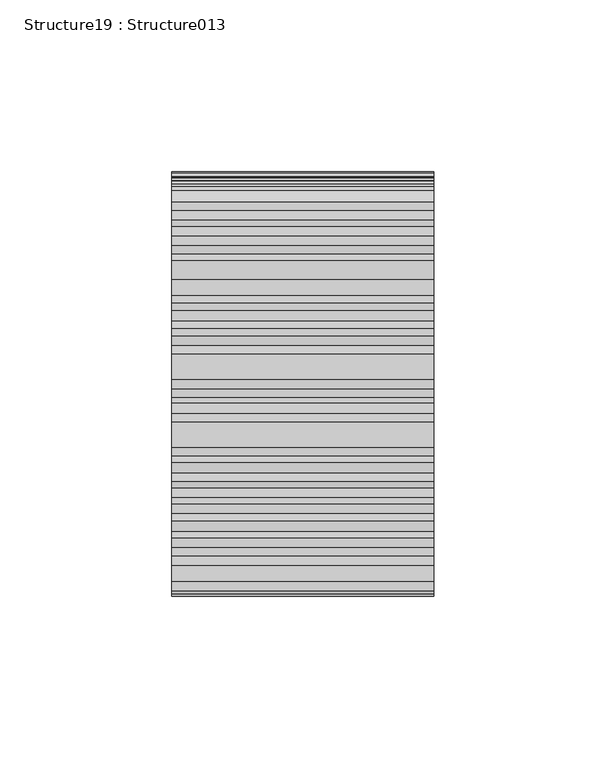
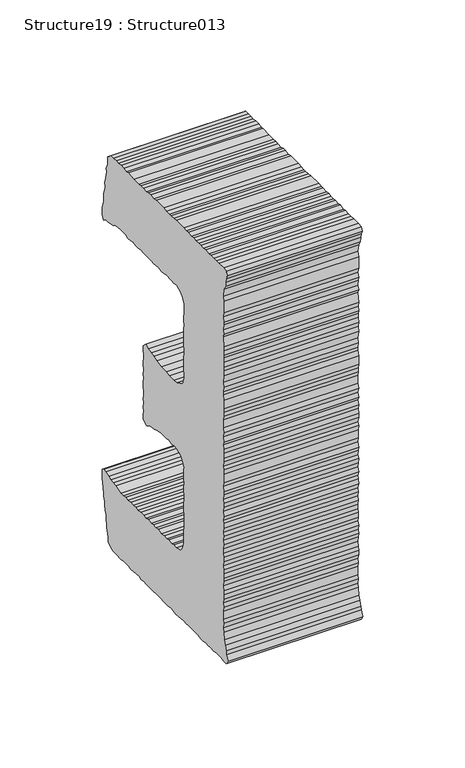
"""IFC4 building model written with IfcOpenShell, lengths in millimetres: proxy geometry, Structure19 : Structure013."""

from ifc_helpers import new_model, si_unit, frame, origin, place, context, project, spatial, polyline, outline, extrude, source, transform, mapped, element, save


def structure19_structure013_5d5198df(model_context):
    return source(origin(), model_context, "Body", "SweptSolid", [
        extrude(outline(polyline([(3.520981, 0.0), (5.3687336, -0.6528764), (7.3730967, -2.6179514), (11.6549807, -5.1627133), (12.9785054, -6.9870238), (17.377171, -10.4155139), (19.218173, -11.0577579), (21.470001, -13.2028271), (23.2331492, -14.9798898), (25.1815783, -16.4985708), (27.2738182, -17.3366394), (28.8385579, -19.3489622), (30.9822906, -20.6170736), (36.8382689, -25.1814496), (38.1096325, -26.5751964), (42.0165135, -29.6203706), (44.5911834, -30.8344637), (46.1186982, -32.4149751), (48.0677955, -33.9341769), (50.0628041, -35.8919606), (51.7241068, -36.7840474), (54.1128276, -38.2560015), (55.8106871, -39.5793789), (59.8256633, -43.5015108), (61.728181, -44.5816098), (63.4819747, -46.3513813), (71.045167, -52.246426), (73.3879764, -53.2797981), (75.3370737, -54.799), (76.9104998, -56.8180933), (78.8043313, -57.8914219), (80.5574566, -59.6606725), (83.2029967, -61.3199119), (84.7155754, -62.9016711), (88.6131018, -65.9395539), (91.0080723, -67.4034897), (92.965856, -68.9294621), (92.6643144, -71.8244284), (89.5384075, -73.3267912), (87.9623774, -74.8320199), (85.5169555, -76.4576858), (83.2585045, -77.843473), (80.1048617, -80.8752535), (78.3434032, -82.6376749), (76.8779249, -85.0153313), (75.2977083, -86.5452241), (72.2514925, -90.4534414), (70.9755889, -92.5878782), (69.2141305, -94.3502996), (68.1882757, -96.6807082), (66.4732494, -98.8810433), (64.89774, -100.3856037), (62.9357699, -102.4052765), (61.4702915, -104.7829329), (60.3813387, -106.6968098), (58.6136505, -108.4479307), (57.3439767, -110.593668), (55.5215234, -111.9175662), (54.245099, -114.0526712), (52.5358016, -116.2456562), (50.958189, -117.7722081), (49.4379456, -119.7226417), (47.9724673, -122.100298), (46.2052799, -123.8700695), (44.9262515, -126.0085154), (43.3486389, -127.5350673), (42.1311261, -130.1113683), (40.1738632, -132.1057087), (38.7827005, -133.3930501), (37.7573665, -135.7227906), (35.5500349, -137.5404779), (34.2710064, -139.6789238), (32.8154035, -142.0632034), (31.1820041, -143.1445502), (29.707672, -145.5335657), (28.6359059, -147.4253925), (26.4207621, -149.2531025), (25.1448585, -151.3875394), (22.1043716, -155.2884067), (20.642519, -157.6807045), (19.0065156, -158.7653922), (17.5968241, -161.5882536), (16.2713635, -163.2887859), (14.3000387, -165.3011673), (13.0329689, -167.4435637), (11.0303155, -168.998654), (10.3716315, -170.8579919), (8.1700287, -172.6683292), (6.9499119, -175.247971), (4.9384047, -176.8144206), (1.892189, -180.7226379), (0.8022144, -182.6185325), (-0.715425, -184.5656252), (-1.7955241, -186.468143), (-5.0360019, -190.6255935), (-7.2344797, -192.4319216), (-8.3708865, -193.8899026), (-9.8446977, -196.2782499), (-11.8009389, -198.2905726), (-13.9710127, -202.088985), (-15.9277547, -204.0826572), (-17.2026366, -206.2350764), (-19.1604203, -208.230085), (-20.680143, -210.1798505), (-21.5800419, -211.851176), (-23.350855, -213.6063061), (-24.6257369, -215.7587252), (-28.5309081, -219.7546975), (-29.1838632, -221.6066852), (-31.1927663, -223.1697939), (-32.8525067, -225.7966834), (-33.7466767, -227.460659), (-35.9540084, -229.2783463), (-37.1689171, -231.8513063), (-41.3562268, -237.2235181), (-43.5541839, -239.0291781), (-45.7331114, -242.8389496), (-46.2144997, -245.9825696), (-47.6804988, -248.3608942), (-48.7141658, -250.7013256), (-49.3210421, -252.9737656), (-51.376024, -254.116422), (-53.782285, -252.6490565), (-57.4392645, -249.7986652), (-59.431001, -247.8380614), (-61.3800983, -246.3188596), (-63.7870274, -244.8509733), (-65.0457643, -243.4616977), (-67.8710036, -242.0523009), (-69.1938602, -240.2285113), (-71.5914347, -238.7679163), (-73.058102, -237.6247391), (-75.0498385, -235.6641353), (-76.8915087, -235.0213703), (-78.4649349, -233.0022771), (-81.2901742, -231.5928803), (-82.5703917, -230.2104926), (-84.7052706, -228.9310221), (-90.5612489, -224.3666461), (-92.3238963, -222.6082338), (-94.5762251, -220.4445143), (-95.7823, -219.5044528), (-97.9386595, -218.2318701), (-100.3241081, -216.7570959), (-106.1800864, -212.1927199), (-107.7448261, -210.1803973), (-110.3288505, -208.9590127), (-112.02671, -207.6356353), (-113.3595894, -205.8040335), (-115.7998031, -203.9020366), (-117.6962384, -202.8320489), (-119.2155677, -201.2396576), (-122.871879, -198.3897871), (-127.6455475, -195.4617092), (-128.7278573, -193.8254111), (-131.0606439, -192.799851), (-133.2603108, -191.0853455), (-135.2735277, -189.1316297), (-136.9166221, -188.235475), (-138.9298392, -186.2817591), (-140.8789365, -184.7625573), (-141.7905737, -180.8994358), (-140.6489589, -179.434773), (-139.1287155, -177.4843394), (-138.2016013, -174.2842644), (-136.6297175, -172.7650626), (-135.7267138, -171.1090466), (-134.9519493, -168.5840025), (-133.5235485, -165.7757238), (-131.9511441, -164.2558538), (-131.1122599, -162.1653238), (-130.0661135, -159.8281746), (-128.7437778, -158.1316514), (-127.2793211, -155.7360128), (-126.3784004, -154.0826695), (-125.4053749, -151.3211764), (-124.316422, -149.4072996), (-122.7966994, -147.4575341), (-119.9900088, -146.9007885), (-119.5437951, -148.8157327), (-117.5295565, -150.787431), (-115.957152, -152.7885418), (-114.2028375, -154.5576451), (-113.7471219, -156.4810696), (-109.7244809, -160.3919897), (-105.8269546, -163.4298725), (-103.7336931, -164.2859234), (-101.544049, -165.9926167), (-99.9616218, -168.0015398), (-97.6364999, -169.0383116), (-95.9386403, -170.361689), (-94.356213, -172.3706122), (-91.7283605, -174.0332513), (-85.8723823, -178.5976272), (-83.7348993, -179.8737569), (-82.027017, -181.2049464), (-80.2040429, -183.4013611), (-78.120136, -184.2501205), (-75.8683081, -186.3951897), (-74.5986342, -187.7704334), (-70.6910851, -190.8161284), (-68.5463307, -192.1022221), (-66.5429891, -194.0493148), (-62.4222757, -195.3083994), (-59.6266295, -194.7258594), (-56.5075132, -193.2515016), (-53.0857937, -188.8615225), (-52.1827898, -187.2055066), (-50.7178323, -184.8285184), (-48.5146472, -182.9968579), (-48.0497244, -181.4054037), (-46.2804537, -179.6329596), (-44.5732396, -177.4426473), (-43.1082822, -175.0656591), (-41.7682389, -173.3464177), (-39.7692111, -171.7766859), (-38.4437505, -170.0761536), (-37.2054253, -167.4924439), (-35.8830896, -165.7959208), (-33.9268483, -163.7835981), (-32.6478199, -161.6451521), (-30.6477505, -160.074084), (-29.4983236, -158.5993985), (-27.8723429, -153.9859176), (-30.5461268, -148.3830343), (-32.791705, -146.2299469), (-36.2068014, -143.5680887), (-39.0387914, -142.1480597), (-42.9363178, -139.1101768), (-46.9248256, -137.1839909), (-49.9365148, -136.0138045), (-52.0192327, -135.1648976), (-54.5939026, -133.9508045), (-57.3096117, -133.3958531), (-57.9216431, -130.1626079), (-57.0358061, -128.5093234), (-53.4983265, -124.9850902), (-51.8437943, -122.3648825), (-50.9438953, -120.6935569), (-48.9412418, -119.1384665), (-47.2804599, -116.5102406), (-45.898151, -115.2342583), (-44.6738677, -112.6492709), (-42.9676951, -110.460295), (-40.9499382, -108.8858273), (-39.4302156, -106.9360618), (-38.3319081, -105.0294762), (-36.7683574, -103.5209654), (-35.5534487, -100.9480054), (-33.7221416, -99.6127481), (-32.446238, -97.4783112), (-30.7369406, -95.2853262), (-27.1561339, -95.7046781), (-26.2070912, -98.0287327), (-24.8816306, -99.8491814), (-22.8198782, -102.2188195), (-21.4410875, -104.4890032), (-18.3462289, -108.0784965), (-16.4523976, -109.1518251), (-14.2074876, -111.3043916), (-12.9298741, -112.6901201), (-10.1046347, -114.099517), (-8.6020789, -115.673464), (-6.3930574, -117.3952608), (-2.2640111, -118.6436543), (-0.7706294, -118.2394317), (3.3944529, -116.398803), (4.0619707, -114.5474246), (6.1963289, -112.3065825), (7.7165723, -110.3561489), (9.2973097, -108.8255879), (10.1372155, -106.7530401), (11.6626671, -104.7959246), (13.8601233, -102.9716141), (15.3803667, -101.0211805), (16.2807666, -99.3685055), (19.1316787, -95.7108577), (21.0853159, -93.7018759), (25.6512543, -87.8438931), (26.5516542, -86.191218), (28.0171324, -83.8135616), (31.2524021, -79.6627929), (32.5539984, -75.9629739), (32.7250243, -73.753612), (29.8254694, -69.9135492), (27.6810685, -68.644917), (26.599427, -67.0091396), (23.7741875, -65.5997428), (22.6918778, -63.9634446), (20.5543948, -62.687315), (18.5531364, -60.7375495), (15.7185424, -59.3208614), (14.1544709, -57.3090594), (12.0163197, -56.0324089), (10.4974913, -54.4586681), (7.914135, -53.2378044), (6.5906103, -51.4134939), (4.6943423, -50.3253765), (2.3087264, -48.8687321), (0.2428475, -46.465802), (-1.6534205, -45.3776847), (-3.4041093, -43.6232228), (-5.5057038, -42.7778629), (-7.5615598, -40.3827451), (-9.4125848, -39.7326888), (-10.9766563, -37.7208868), (-12.9257535, -36.201685), (-17.6008287, -34.1420845), (-19.7368967, -32.8627613), (-21.8286158, -32.0240246), (-24.1014292, -31.4190054), (-26.9328983, -29.9983082), (-28.5176019, -29.5440175), (-29.2337625, -27.4186663), (-27.3291615, -24.9751117), (-25.8115221, -23.028019), (-24.1755187, -21.9433312), (-22.0321594, -19.6923188), (-19.7695618, -18.3205047), (-18.6894627, -16.417987), (-16.374704, -15.4767366), (-15.099822, -13.3243174), (-12.9013442, -11.5179892), (-10.8465097, -10.3741438), (-8.9450335, -7.9345983), (-7.1225803, -6.6107002), (-5.7919115, -4.9034861), (-3.5322715, -3.5175514), (-1.3947885, -1.2727), (0.0, 0.0), (3.520981, 0.0)])), frame((-35624.0862846, 276992.6835133, 3985.6060189), z_axis=(1.0, 0.0, 1.354250045437766e-12), x_axis=(0.0, -0.7887169572514444, -0.6147565057354197)), (0.0, 0.0, 1.0), 76.2),
    ])


if __name__ == "__main__":
    model = new_model("IFC4")
    model_context = context("Model", 3, world=origin())
    ifc_project = project(units=[si_unit("LENGTHUNIT", "METRE", prefix="MILLI")], contexts=[model_context])
    site = spatial("IfcSite", under=ifc_project)
    building = spatial("IfcBuilding", under=site)
    placement = place(None, origin())
    structure19_structure013_shape = structure19_structure013_5d5198df(model_context)
    element("IfcBuildingElementProxy", 1, Name="Structure19 : Structure013", ObjectType="Structure19 : Structure013", at=placement, inside=building, context=model_context, shape_type="MappedRepresentation", body=[
        mapped(structure19_structure013_shape, transform((0.0, 0.0, 0.0), x_axis=(1.0, 0.0, 0.0), y_axis=(0.0, 1.0, 0.0), z_axis=(0.0, 0.0, 1.0))),
    ])
    save(model, "model.ifc")

# Revit data of these elements
# Type "Structure19 : Structure013"
#   NameOverride = "Structure013"
# Element 1 (IfcBuildingElementProxy, "Structure19 : Structure013")
#   Materials on its faces: "BRUSHED ALUMINUM LETTERING"
# Materials
#   "BRUSHED ALUMINUM LETTERING": class "Unassigned", colour RGB 169 181 186, transparency 0, Cost = 0
